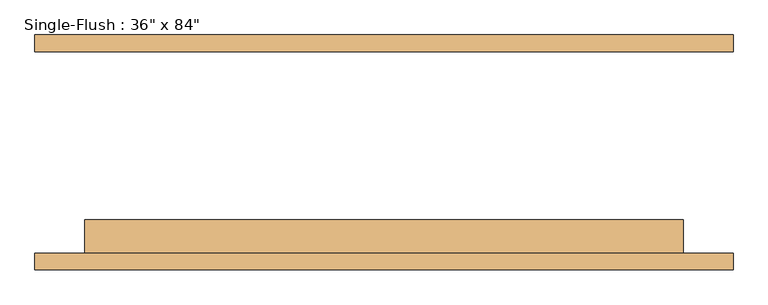
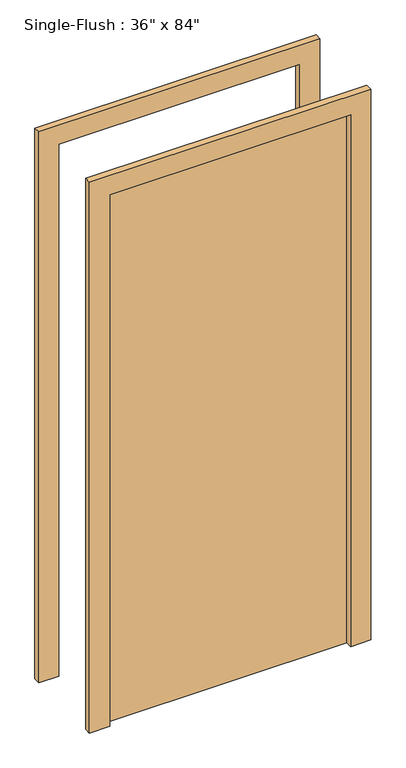
"""IFC4 building model written with IfcOpenShell, lengths in millimetres: door geometry."""

from ifc_helpers import new_model, si_unit, frame, origin, origin_with_axes, place, context, project, spatial, polyline, outline, extrude, source, transform, mapped, element, save


def door_90af15fc(model_context):
    return source(origin(), model_context, "Body", "SweptSolid", [
        extrude(outline(polyline([(2209.8, -533.4), (0.0, -533.4), (0.0, -457.2), (2133.6, -457.2), (2133.6, 457.2), (0.0, 457.2), (0.0, 533.4), (2209.8, 533.4), (2209.8, -533.4)])), frame((0.0, -179.3875, 0.0), z_axis=(0.0, 1.0, 0.0), x_axis=(0.0, 0.0, 1.0)), (0.0, 0.0, 1.0), 25.4),
        extrude(outline(polyline([(2209.8, 533.4), (2209.8, -533.4), (0.0, -533.4), (0.0, -457.2), (2133.6, -457.2), (2133.6, 457.2), (0.0, 457.2), (0.0, 533.4), (2209.8, 533.4)])), frame((0.0, 153.9875, 0.0), z_axis=(0.0, 1.0, 0.0), x_axis=(0.0, 0.0, 1.0)), (0.0, 0.0, 1.0), 25.4),
        extrude(outline(polyline([(457.2, -103.1875), (457.2, -153.9875), (-457.2, -153.9875), (-457.2, -103.1875), (457.2, -103.1875)])), origin_with_axes(), (0.0, 0.0, 1.0), 2133.6),
    ])


if __name__ == "__main__":
    model = new_model("IFC4")
    model_context = context("Model", 3, world=origin())
    ifc_project = project(units=[si_unit("LENGTHUNIT", "METRE", prefix="MILLI")], contexts=[model_context])
    site = spatial("IfcSite", under=ifc_project)
    building = spatial("IfcBuilding", under=site)
    placement = place(None, origin())
    door_shape = door_90af15fc(model_context)
    element("IfcDoor", 1, ObjectType="Single-Flush : 36\" x 84\"", at=placement, inside=building, context=model_context, shape_type="MappedRepresentation", body=[
        mapped(door_shape, transform((0.0, 0.0, 0.0), x_axis=(1.0, 0.0, 0.0), y_axis=(0.0, 1.0, 0.0), z_axis=(0.0, 0.0, 1.0))),
    ])
    save(model, "model.ifc")

# Revit data of these elements
# Type "Single-Flush : 36\" x 84\""
#   Type Mark = "1"
#   Assembly Code = "C1020"
#   Thickness = 0' - 2"
#   Height = 7' - 0"
#   Trim Projection Ext = 0' - 1"
#   Trim Projection Int = 0' - 1"
#   Trim Width = 0' - 3"
#   Width = 3' - 0"
#   Function = 0
#   Door Material = Door - Panel
#   Frame Material = Door - Frame
#   Wall Closure = (empty or 0)
# Element 1 (IfcDoor, "Single-Flush : 36\" x 84\"")
#   Materials on its faces: "Door - Frame", "Door - Panel"
# Materials
#   "Door - Panel": class "Wood", colour RGB 210 159 95, transparency 0
#   "Door - Frame": class "Miscellaneous", colour RGB 118 70 51, transparency 0
